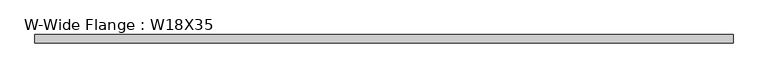
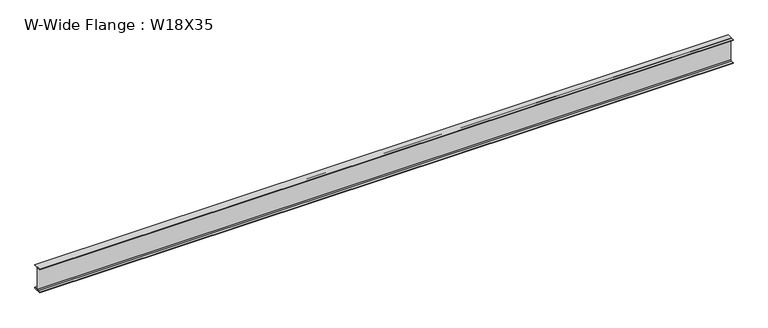
"""IFC4 building model written with IfcOpenShell, lengths in millimetres: beam geometry, W-Wide Flange : W18X35."""

from ifc_helpers import new_model, si_unit, point, frame, frame_2d, origin, place, context, project, spatial, polyline, circle_curve, trimmed, segment, composite_curve, outline, extrude, source, transform, mapped, element, save


def w_wide_flange_w18x35_c138c6e5(model_context):
    return source(origin(), model_context, "Body", "SweptSolid", [
        extrude(outline(composite_curve([segment(polyline([(76.2, -213.995), (76.2, -224.79), (-76.2, -224.79), (-76.2, -213.995), (-21.59, -213.995)]), True, "CONTINUOUS"), segment(trimmed(circle_curve(frame_2d((-21.59, -196.215)), 17.78), [point((-21.59, -213.995))], [point((-3.81, -196.215))], True, "CARTESIAN"), True, "CONTINUOUS"), segment(polyline([(-3.81, -196.215), (-3.81, 196.215)]), True, "CONTINUOUS"), segment(trimmed(circle_curve(frame_2d((-21.59, 196.215)), 17.78), [point((-3.81, 196.215))], [point((-21.59, 213.995))], True, "CARTESIAN"), True, "CONTINUOUS"), segment(polyline([(-21.59, 213.995), (-76.2, 213.995), (-76.2, 224.79), (76.2, 224.79), (76.2, 213.995), (21.59, 213.995)]), True, "CONTINUOUS"), segment(trimmed(circle_curve(frame_2d((21.59, 196.215)), 17.78), [point((21.59, 213.995))], [point((3.81, 196.215))], True, "CARTESIAN"), True, "CONTINUOUS"), segment(polyline([(3.81, 196.215), (3.81, -196.215)]), True, "CONTINUOUS"), segment(trimmed(circle_curve(frame_2d((21.59, -196.215)), 17.78), [point((3.81, -196.215))], [point((21.59, -213.995))], True, "CARTESIAN"), True, "CONTINUOUS"), segment(polyline([(21.59, -213.995), (76.2, -213.995)]), True, "CONTINUOUS")], self_intersect=False)), frame((-6252.4306073, 0.0, 0.0), z_axis=(1.0, 0.0, 0.0), x_axis=(0.0, 1.0, 0.0)), (0.0, 0.0, 1.0), 12515.3685994),
    ])


if __name__ == "__main__":
    model = new_model("IFC4")
    model_context = context("Model", 3, world=origin())
    ifc_project = project(units=[si_unit("LENGTHUNIT", "METRE", prefix="MILLI")], contexts=[model_context])
    site = spatial("IfcSite", under=ifc_project)
    building = spatial("IfcBuilding", under=site)
    placement = place(None, origin())
    w_wide_flange_w18x35_shape = w_wide_flange_w18x35_c138c6e5(model_context)
    element("IfcBeam", 1, ObjectType="W-Wide Flange : W18X35", at=placement, inside=building, context=model_context, shape_type="MappedRepresentation", body=[
        mapped(w_wide_flange_w18x35_shape, transform((0.0, 0.0, 0.0), x_axis=(1.0, 0.0, 0.0), y_axis=(0.0, 1.0, 0.0), z_axis=(0.0, 0.0, 1.0))),
    ])
    save(model, "model.ifc")

# Revit data of these elements
# Type "W-Wide Flange : W18X35"
#   Assembly Code = "B10"
#   W = 35
#   Length [instance default] = 5' - 0"
#   bf = 0' - 6"
#   d = 1' - 5.7"
#   k = 0' - 1 1/8"
#   k2 = 0' - 0.7"
#   tf = 0' - 0.425"
#   tw = 0' - 0.3"
#   A = 0.0715278 SF
#   Structural Material [instance default] = Steel ASTM A992
# Element 1 (IfcBeam, "W-Wide Flange : W18X35")
#   Structural Material = Steel ASTM A36
#   Materials on its faces: "Steel ASTM A36"
# Materials
#   "Steel ASTM A992": class "Metal", colour RGB 199 199 199, transparency 0, Description = "Structural steel 50ksi", Cost = 0
#   "Steel ASTM A36": class "Metal", colour RGB 199 199 199, transparency 0, Description = "Structural steel, ASTM A36 Grade B, mill finish", Cost = 0
